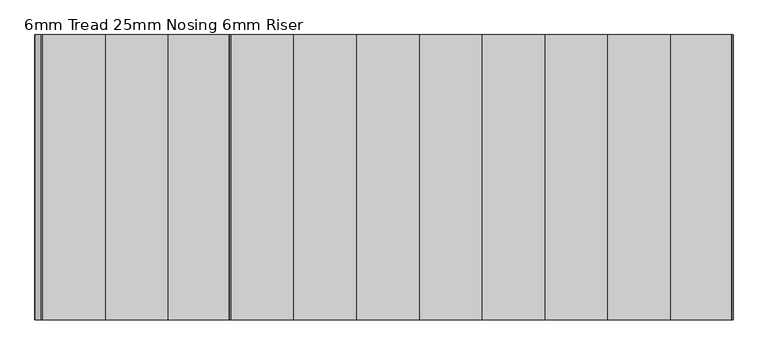
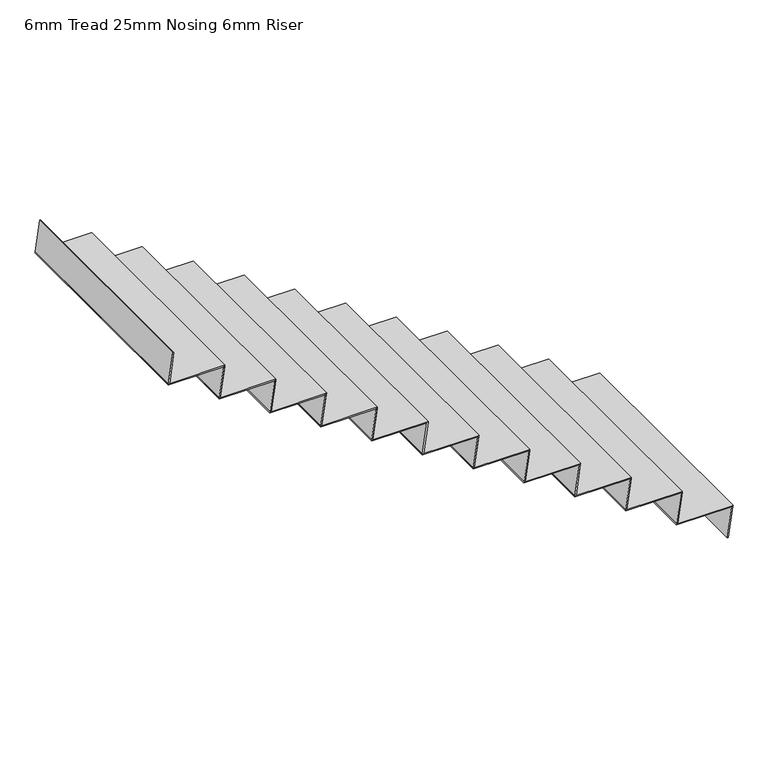
"""IFC4 building model written with IfcOpenShell, lengths in millimetres: stair flight geometry, 6mm Tread 25mm Nosing 6mm Riser."""

from ifc_helpers import new_model, si_unit, origin, place, context, project, spatial, faceted_brep, source, transform, mapped, element, save


def stair_flight_6mm_tread_25mm_nosing_6mm_riser_b549f667(model_context):
    return source(origin(), model_context, "Body", "Brep", [
        faceted_brep([(-13631.0599092, 11470.4345331, 16470.5882353), (-13631.9099092, 11470.4345331, 16464.5882353), (-13631.9099092, 10220.4345331, 16464.5882353), (-13631.0599092, 10220.4345331, 16470.5882353), (-13325.0, 10220.4345331, 16470.5882353), (-13325.0, 11470.4345331, 16470.5882353), (-13325.85, 11470.4345331, 16464.5882353), (-13325.85, 10220.4345331, 16464.5882353)], [[[0, 1, 2, 3]], [[3, 4, 5, 0]], [[2, 1, 6, 7]], [[4, 3, 2, 7]], [[0, 5, 6, 1]], [[5, 4, 7, 6]]]),
        faceted_brep([(-13325.85, 11470.4345331, 16464.5882353), (-13350.0, 11470.4345331, 16294.1176471), (-13356.0599092, 11470.4345331, 16294.1176471), (-13331.9099092, 11470.4345331, 16464.5882353), (-13325.85, 10220.4345331, 16464.5882353), (-13331.9099092, 10220.4345331, 16464.5882353), (-13356.0599092, 10220.4345331, 16294.1176471), (-13350.0, 10220.4345331, 16294.1176471)], [[[0, 1, 2, 3]], [[4, 5, 6, 7]], [[1, 0, 4, 7]], [[2, 1, 7, 6]], [[3, 2, 6, 5]], [[0, 3, 5, 4]]]),
        faceted_brep([(-13600.85, 11470.4345331, 16641.0588235), (-13625.0, 11470.4345331, 16470.5882353), (-13631.0599092, 11470.4345331, 16470.5882353), (-13606.9099092, 11470.4345331, 16641.0588235), (-13600.85, 10220.4345331, 16641.0588235), (-13606.9099092, 10220.4345331, 16641.0588235), (-13631.0599092, 10220.4345331, 16470.5882353), (-13625.0, 10220.4345331, 16470.5882353)], [[[0, 1, 2, 3]], [[4, 5, 6, 7]], [[1, 0, 4, 7]], [[2, 1, 7, 6]], [[3, 2, 6, 5]], [[0, 3, 5, 4]]]),
        faceted_brep([(-13906.0599092, 10220.4345331, 16647.0588235), (-13600.0, 10220.4345331, 16647.0588235), (-13600.0, 11470.4345331, 16647.0588235), (-13906.0599092, 11470.4345331, 16647.0588235), (-13906.9099092, 10220.4345331, 16641.0588235), (-13906.9099092, 11470.4345331, 16641.0588235), (-13600.85, 11470.4345331, 16641.0588235), (-13600.85, 10220.4345331, 16641.0588235)], [[[0, 1, 2, 3]], [[4, 5, 6, 7]], [[1, 0, 4, 7]], [[3, 2, 6, 5]], [[3, 5, 4, 0]], [[2, 1, 7, 6]]]),
        faceted_brep([(-13875.85, 11470.4345331, 16817.5294118), (-13900.0, 11470.4345331, 16647.0588235), (-13906.0599092, 11470.4345331, 16647.0588235), (-13881.9099092, 11470.4345331, 16817.5294118), (-13875.85, 10220.4345331, 16817.5294118), (-13881.9099092, 10220.4345331, 16817.5294118), (-13906.0599092, 10220.4345331, 16647.0588235), (-13900.0, 10220.4345331, 16647.0588235)], [[[0, 1, 2, 3]], [[4, 5, 6, 7]], [[1, 0, 4, 7]], [[2, 1, 7, 6]], [[3, 2, 6, 5]], [[0, 3, 5, 4]]]),
        faceted_brep([(-14181.0599092, 10220.4345331, 16823.5294118), (-13875.0, 10220.4345331, 16823.5294118), (-13875.0, 11470.4345331, 16823.5294118), (-14181.0599092, 11470.4345331, 16823.5294118), (-14181.9099092, 10220.4345331, 16817.5294118), (-14181.9099092, 11470.4345331, 16817.5294118), (-13875.85, 11470.4345331, 16817.5294118), (-13875.85, 10220.4345331, 16817.5294118)], [[[0, 1, 2, 3]], [[4, 5, 6, 7]], [[1, 0, 4, 7]], [[3, 2, 6, 5]], [[3, 5, 4, 0]], [[2, 1, 7, 6]]]),
        faceted_brep([(-14150.85, 11470.4345331, 16994.0), (-14175.0, 11470.4345331, 16823.5294118), (-14181.0599092, 11470.4345331, 16823.5294118), (-14156.9099092, 11470.4345331, 16994.0), (-14150.85, 10220.4345331, 16994.0), (-14156.9099092, 10220.4345331, 16994.0), (-14181.0599092, 10220.4345331, 16823.5294118), (-14175.0, 10220.4345331, 16823.5294118)], [[[0, 1, 2, 3]], [[4, 5, 6, 7]], [[1, 0, 4, 7]], [[2, 1, 7, 6]], [[3, 2, 6, 5]], [[0, 3, 5, 4]]]),
        faceted_brep([(-14456.0599092, 10220.4345331, 17000.0), (-14150.0, 10220.4345331, 17000.0), (-14150.0, 11470.4345331, 17000.0), (-14456.0599092, 11470.4345331, 17000.0), (-14456.9099092, 10220.4345331, 16994.0), (-14456.9099092, 11470.4345331, 16994.0), (-14150.85, 11470.4345331, 16994.0), (-14150.85, 10220.4345331, 16994.0)], [[[0, 1, 2, 3]], [[4, 5, 6, 7]], [[1, 0, 4, 7]], [[3, 2, 6, 5]], [[3, 5, 4, 0]], [[2, 1, 7, 6]]]),
        faceted_brep([(-14425.85, 11470.4345331, 17170.4705882), (-14450.0, 11470.4345331, 17000.0), (-14456.0599092, 11470.4345331, 17000.0), (-14431.9099092, 11470.4345331, 17170.4705882), (-14425.85, 10220.4345331, 17170.4705882), (-14431.9099092, 10220.4345331, 17170.4705882), (-14456.0599092, 10220.4345331, 17000.0), (-14450.0, 10220.4345331, 17000.0)], [[[0, 1, 2, 3]], [[4, 5, 6, 7]], [[1, 0, 4, 7]], [[2, 1, 7, 6]], [[3, 2, 6, 5]], [[0, 3, 5, 4]]]),
        faceted_brep([(-14731.0599092, 10220.4345331, 17176.4705882), (-14425.0, 10220.4345331, 17176.4705882), (-14425.0, 11470.4345331, 17176.4705882), (-14731.0599092, 11470.4345331, 17176.4705882), (-14731.9099092, 10220.4345331, 17170.4705882), (-14731.9099092, 11470.4345331, 17170.4705882), (-14425.85, 11470.4345331, 17170.4705882), (-14425.85, 10220.4345331, 17170.4705882)], [[[0, 1, 2, 3]], [[4, 5, 6, 7]], [[1, 0, 4, 7]], [[3, 2, 6, 5]], [[3, 5, 4, 0]], [[2, 1, 7, 6]]]),
        faceted_brep([(-14700.85, 11470.4345331, 17346.9411765), (-14725.0, 11470.4345331, 17176.4705882), (-14731.0599092, 11470.4345331, 17176.4705882), (-14706.9099092, 11470.4345331, 17346.9411765), (-14700.85, 10220.4345331, 17346.9411765), (-14706.9099092, 10220.4345331, 17346.9411765), (-14731.0599092, 10220.4345331, 17176.4705882), (-14725.0, 10220.4345331, 17176.4705882)], [[[0, 1, 2, 3]], [[4, 5, 6, 7]], [[1, 0, 4, 7]], [[2, 1, 7, 6]], [[3, 2, 6, 5]], [[0, 3, 5, 4]]]),
        faceted_brep([(-15006.0599092, 10220.4345331, 17352.9411765), (-14700.0, 10220.4345331, 17352.9411765), (-14700.0, 11470.4345331, 17352.9411765), (-15006.0599092, 11470.4345331, 17352.9411765), (-15006.9099092, 10220.4345331, 17346.9411765), (-15006.9099092, 11470.4345331, 17346.9411765), (-14700.85, 11470.4345331, 17346.9411765), (-14700.85, 10220.4345331, 17346.9411765)], [[[0, 1, 2, 3]], [[4, 5, 6, 7]], [[1, 0, 4, 7]], [[3, 2, 6, 5]], [[3, 5, 4, 0]], [[2, 1, 7, 6]]]),
        faceted_brep([(-14975.85, 11470.4345331, 17523.4117647), (-15000.0, 11470.4345331, 17352.9411765), (-15006.0599092, 11470.4345331, 17352.9411765), (-14981.9099092, 11470.4345331, 17523.4117647), (-14975.85, 10220.4345331, 17523.4117647), (-14981.9099092, 10220.4345331, 17523.4117647), (-15006.0599092, 10220.4345331, 17352.9411765), (-15000.0, 10220.4345331, 17352.9411765)], [[[0, 1, 2, 3]], [[4, 5, 6, 7]], [[1, 0, 4, 7]], [[2, 1, 7, 6]], [[3, 2, 6, 5]], [[0, 3, 5, 4]]]),
        faceted_brep([(-15281.0599092, 10220.4345331, 17529.4117647), (-14975.0, 10220.4345331, 17529.4117647), (-14975.0, 11470.4345331, 17529.4117647), (-15281.0599092, 11470.4345331, 17529.4117647), (-15281.9099092, 10220.4345331, 17523.4117647), (-15281.9099092, 11470.4345331, 17523.4117647), (-14975.85, 11470.4345331, 17523.4117647), (-14975.85, 10220.4345331, 17523.4117647)], [[[0, 1, 2, 3]], [[4, 5, 6, 7]], [[1, 0, 4, 7]], [[3, 2, 6, 5]], [[3, 5, 4, 0]], [[2, 1, 7, 6]]]),
        faceted_brep([(-15250.85, 11470.4345331, 17699.8823529), (-15275.0, 11470.4345331, 17529.4117647), (-15281.0599092, 11470.4345331, 17529.4117647), (-15256.9099092, 11470.4345331, 17699.8823529), (-15250.85, 10220.4345331, 17699.8823529), (-15256.9099092, 10220.4345331, 17699.8823529), (-15281.0599092, 10220.4345331, 17529.4117647), (-15275.0, 10220.4345331, 17529.4117647)], [[[0, 1, 2, 3]], [[4, 5, 6, 7]], [[1, 0, 4, 7]], [[2, 1, 7, 6]], [[3, 2, 6, 5]], [[0, 3, 5, 4]]]),
        faceted_brep([(-15556.0599092, 10220.4345331, 17705.8823529), (-15250.0, 10220.4345331, 17705.8823529), (-15250.0, 11470.4345331, 17705.8823529), (-15556.0599092, 11470.4345331, 17705.8823529), (-15556.9099092, 10220.4345331, 17699.8823529), (-15556.9099092, 11470.4345331, 17699.8823529), (-15250.85, 11470.4345331, 17699.8823529), (-15250.85, 10220.4345331, 17699.8823529)], [[[0, 1, 2, 3]], [[4, 5, 6, 7]], [[1, 0, 4, 7]], [[3, 2, 6, 5]], [[3, 5, 4, 0]], [[2, 1, 7, 6]]]),
        faceted_brep([(-15525.85, 11470.4345331, 17876.3529412), (-15550.0, 11470.4345331, 17705.8823529), (-15556.0599092, 11470.4345331, 17705.8823529), (-15531.9099092, 11470.4345331, 17876.3529412), (-15525.85, 10220.4345331, 17876.3529412), (-15531.9099092, 10220.4345331, 17876.3529412), (-15556.0599092, 10220.4345331, 17705.8823529), (-15550.0, 10220.4345331, 17705.8823529)], [[[0, 1, 2, 3]], [[4, 5, 6, 7]], [[1, 0, 4, 7]], [[2, 1, 7, 6]], [[3, 2, 6, 5]], [[0, 3, 5, 4]]]),
        faceted_brep([(-15831.0599092, 10220.4345331, 17882.3529412), (-15525.0, 10220.4345331, 17882.3529412), (-15525.0, 11470.4345331, 17882.3529412), (-15831.0599092, 11470.4345331, 17882.3529412), (-15831.9099092, 10220.4345331, 17876.3529412), (-15831.9099092, 11470.4345331, 17876.3529412), (-15525.85, 11470.4345331, 17876.3529412), (-15525.85, 10220.4345331, 17876.3529412)], [[[0, 1, 2, 3]], [[4, 5, 6, 7]], [[1, 0, 4, 7]], [[3, 2, 6, 5]], [[3, 5, 4, 0]], [[2, 1, 7, 6]]]),
        faceted_brep([(-15800.85, 11470.4345331, 18052.8235294), (-15825.0, 11470.4345331, 17882.3529412), (-15831.0599092, 11470.4345331, 17882.3529412), (-15806.9099092, 11470.4345331, 18052.8235294), (-15800.85, 10220.4345331, 18052.8235294), (-15806.9099092, 10220.4345331, 18052.8235294), (-15831.0599092, 10220.4345331, 17882.3529412), (-15825.0, 10220.4345331, 17882.3529412)], [[[0, 1, 2, 3]], [[4, 5, 6, 7]], [[1, 0, 4, 7]], [[2, 1, 7, 6]], [[3, 2, 6, 5]], [[0, 3, 5, 4]]]),
        faceted_brep([(-16106.0599092, 10220.4345331, 18058.8235294), (-15800.0, 10220.4345331, 18058.8235294), (-15800.0, 11470.4345331, 18058.8235294), (-16106.0599092, 11470.4345331, 18058.8235294), (-16106.9099092, 10220.4345331, 18052.8235294), (-16106.9099092, 11470.4345331, 18052.8235294), (-15800.85, 11470.4345331, 18052.8235294), (-15800.85, 10220.4345331, 18052.8235294)], [[[0, 1, 2, 3]], [[4, 5, 6, 7]], [[1, 0, 4, 7]], [[3, 2, 6, 5]], [[3, 5, 4, 0]], [[2, 1, 7, 6]]]),
        faceted_brep([(-16350.85, 11470.4345331, 18405.7647059), (-16375.0, 11470.4345331, 18235.2941176), (-16381.0599092, 11470.4345331, 18235.2941176), (-16356.9099092, 11470.4345331, 18405.7647059), (-16350.85, 10220.4345331, 18405.7647059), (-16356.9099092, 10220.4345331, 18405.7647059), (-16381.0599092, 10220.4345331, 18235.2941176), (-16375.0, 10220.4345331, 18235.2941176)], [[[0, 1, 2, 3]], [[4, 5, 6, 7]], [[1, 0, 4, 7]], [[2, 1, 7, 6]], [[3, 2, 6, 5]], [[0, 3, 5, 4]]]),
        faceted_brep([(-16075.85, 11470.4345331, 18229.2941176), (-16100.0, 11470.4345331, 18058.8235294), (-16106.0599092, 11470.4345331, 18058.8235294), (-16081.9099092, 11470.4345331, 18229.2941176), (-16075.85, 10220.4345331, 18229.2941176), (-16081.9099092, 10220.4345331, 18229.2941176), (-16106.0599092, 10220.4345331, 18058.8235294), (-16100.0, 10220.4345331, 18058.8235294)], [[[0, 1, 2, 3]], [[4, 5, 6, 7]], [[1, 0, 4, 7]], [[2, 1, 7, 6]], [[3, 2, 6, 5]], [[0, 3, 5, 4]]]),
        faceted_brep([(-16381.0599092, 10220.4345331, 18235.2941176), (-16350.0, 10220.4345331, 18235.2941176), (-16075.0, 10220.4345331, 18235.2941176), (-16075.0, 11470.4345331, 18235.2941176), (-16381.0599092, 11470.4345331, 18235.2941176), (-16381.9099092, 10220.4345331, 18229.2941176), (-16381.9099092, 11470.4345331, 18229.2941176), (-16075.85, 11470.4345331, 18229.2941176), (-16075.85, 10220.4345331, 18229.2941176), (-16350.0, 10220.4345331, 18229.2941176)], [[[0, 1, 2, 3, 4]], [[5, 6, 7, 8, 9]], [[1, 0, 5, 9]], [[2, 1, 9, 8]], [[4, 3, 7, 6]], [[4, 6, 5, 0]], [[3, 2, 8, 7]]]),
    ])


if __name__ == "__main__":
    model = new_model("IFC4")
    model_context = context("Model", 3, world=origin())
    ifc_project = project(units=[si_unit("LENGTHUNIT", "METRE", prefix="MILLI")], contexts=[model_context])
    site = spatial("IfcSite", under=ifc_project)
    building = spatial("IfcBuilding", under=site)
    placement = place(None, origin())
    stair_flight_6mm_tread_25mm_nosing_6mm_riser_shape = stair_flight_6mm_tread_25mm_nosing_6mm_riser_b549f667(model_context)
    element("IfcStairFlight", 1, ObjectType="6mm Tread 25mm Nosing 6mm Riser", at=placement, inside=building, context=model_context, shape_type="MappedRepresentation", body=[
        mapped(stair_flight_6mm_tread_25mm_nosing_6mm_riser_shape, transform((0.0, 0.0, 0.0), x_axis=(1.0, 0.0, 0.0), y_axis=(0.0, 1.0, 0.0), z_axis=(0.0, 0.0, 1.0))),
    ])
    save(model, "model.ifc")

# Revit data of these elements
# Element 1 (IfcStairFlight, "6mm Tread 25mm Nosing 6mm Riser")
#   Materials on its faces: "Steel, Paint Finish, Dark Gray"
# Materials
#   "Steel, Paint Finish, Dark Gray": class "Metal", colour RGB 89 89 89, transparency 0, Description = "Steel, paint finish, dark gray, glossy", Cost = 0
